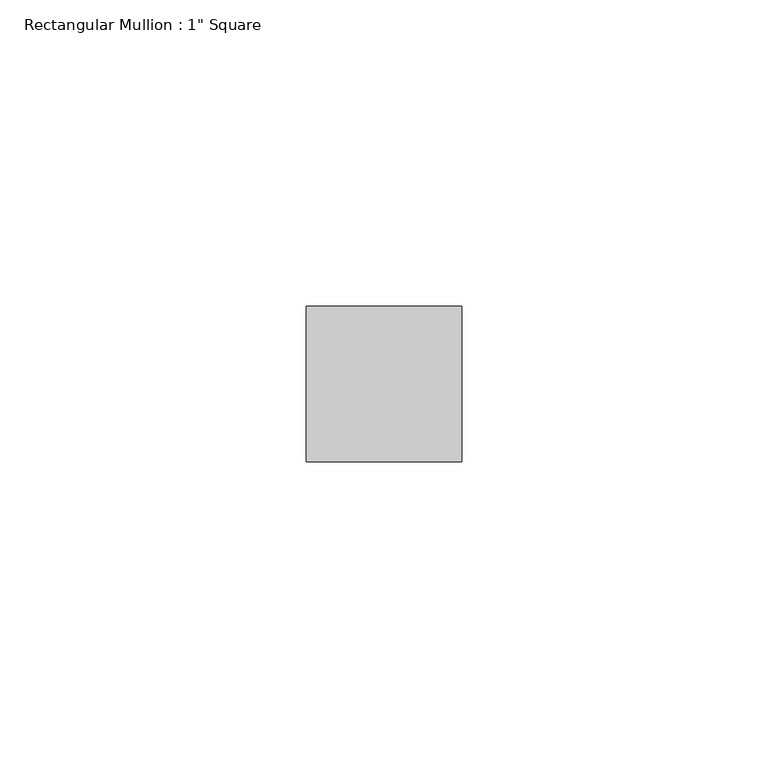
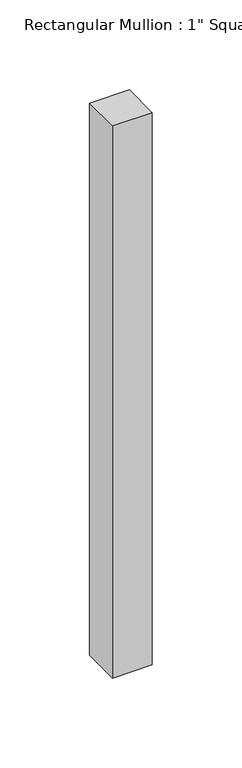
"""IFC4 building model written with IfcOpenShell, lengths in millimetres: member geometry."""

from ifc_helpers import new_model, si_unit, frame, origin, place, context, project, spatial, polyline, outline, extrude, source, transform, mapped, element, save


def member_fdcf86f7(model_context):
    return source(origin(), model_context, "Body", "SweptSolid", [
        extrude(outline(polyline([(12.7, 12.7), (12.7, -12.7), (-12.7, -12.7), (-12.7, 12.7), (12.7, 12.7)])), frame((0.0, 0.0, -374.6499997), z_axis=(0.0, 0.0, 1.0), x_axis=(1.0, 0.0, 0.0)), (0.0, 0.0, 1.0), 374.6499997),
    ])


if __name__ == "__main__":
    model = new_model("IFC4")
    model_context = context("Model", 3, world=origin())
    ifc_project = project(units=[si_unit("LENGTHUNIT", "METRE", prefix="MILLI")], contexts=[model_context])
    site = spatial("IfcSite", under=ifc_project)
    building = spatial("IfcBuilding", under=site)
    placement = place(None, origin())
    member_shape = member_fdcf86f7(model_context)
    element("IfcMember", 1, ObjectType="Rectangular Mullion : 1\" Square", at=placement, inside=building, context=model_context, shape_type="MappedRepresentation", body=[
        mapped(member_shape, transform((0.0, 0.0, 0.0), x_axis=(1.0, 0.0, 0.0), y_axis=(0.0, 1.0, 0.0), z_axis=(0.0, 0.0, 1.0))),
    ])
    save(model, "model.ifc")

# Revit data of these elements
# Type "Rectangular Mullion : 1\" Square"
#   built-in parameter 1007304 = 0.0833333 (stored number, unit not read)
#   built-in parameter 1007301 = 0.0416667 (stored number, unit not read)
#   built-in parameter 1007300 = 0.0416667 (stored number, unit not read)
# Element 1 (IfcMember, "Rectangular Mullion : 1\" Square")
#   Materials on its faces: "Metal - Aluminum"
# Materials
#   "Metal - Aluminum": class "Metal", colour RGB 247 247 247, transparency 0
